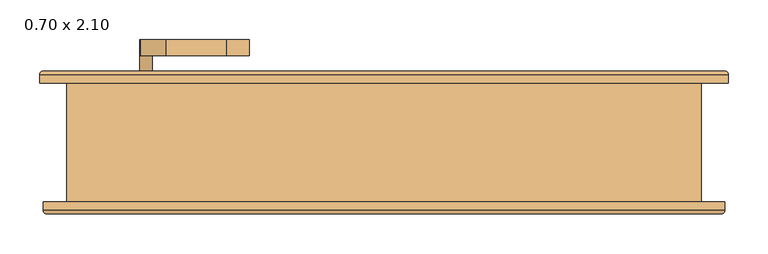
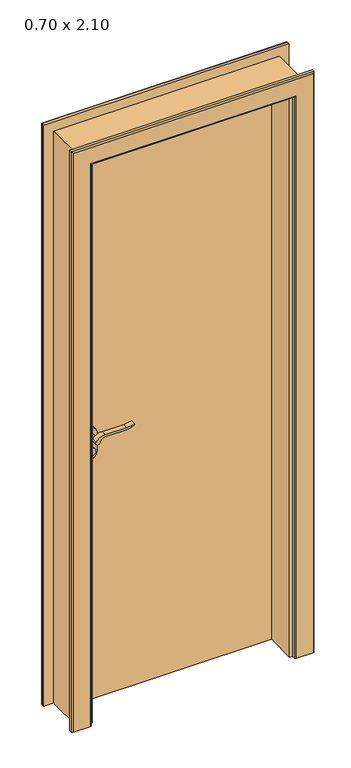
"""IFC4 building model written with IfcOpenShell, lengths in millimetres: door geometry, PORTA_DE_ABRIR_MADEIRA : 0.70 x 2.10."""

from ifc_helpers import new_model, si_unit, point, frame, frame_2d, origin, origin_with_axes, place, context, project, spatial, polyline, circle_curve, ellipse_curve, trimmed, segment, composite_curve, outline, extrude, faceted_brep, source, transform, mapped, element, save
from ifc_brep_helpers import plane_surface, cylinder_surface, advanced_brep


def door_0_70_x_2_10_357bc0c5(model_context):
    return source(origin(), model_context, "Body", "SolidModel", [
        extrude(outline(composite_curve([segment(trimmed(circle_curve(frame_2d((940.0, -300.0)), 15.0), [point((940.0, -285.0))], [point((940.0, -315.0))], False, "CARTESIAN"), True, "CONTINUOUS"), segment(trimmed(circle_curve(frame_2d((940.0, -300.0)), 15.0), [point((940.0, -315.0))], [point((940.0, -285.0))], False, "CARTESIAN"), True, "CONTINUOUS")], self_intersect=False)), frame((0.0, 15.0, 0.0), z_axis=(0.0, 1.0, 0.0), x_axis=(0.0, 0.0, 1.0)), (0.0, 0.0, 1.0), 10.0),
        extrude(outline(composite_curve([segment(trimmed(circle_curve(frame_2d((940.0, -300.0)), 15.0), [point((940.0, -285.0))], [point((940.0, -315.0))], False, "CARTESIAN"), True, "CONTINUOUS"), segment(trimmed(circle_curve(frame_2d((940.0, -300.0)), 15.0), [point((940.0, -315.0))], [point((940.0, -285.0))], False, "CARTESIAN"), True, "CONTINUOUS")], self_intersect=False)), frame((0.0, 80.0, 0.0), z_axis=(0.0, 1.0, 0.0), x_axis=(0.0, 0.0, 1.0)), (0.0, 0.0, 1.0), 10.0),
        extrude(outline(composite_curve([segment(trimmed(circle_curve(frame_2d((1000.0, -300.0)), 8.0), [point((1004.6523287, -306.5081363))], [point((1000.0, -292.0))], False, "CARTESIAN"), True, "CONTINUOUS"), segment(trimmed(circle_curve(frame_2d((994.8738613, -274.6138099)), 18.1261387), [point((1000.0, -292.0))], [point((1013.0, -274.6138099))], True, "CARTESIAN"), True, "CONTINUOUS"), segment(polyline([(1013.0, -274.6138099), (1013.0, -198.3564091)]), True, "CONTINUOUS"), segment(trimmed(circle_curve(frame_2d((1072.2709207, -201.9396612)), 59.3791355), [point((1013.0, -198.3564091))], [point((1022.2135558, -170.0))], False, "CARTESIAN"), True, "CONTINUOUS"), segment(polyline([(1022.2135558, -170.0), (1025.0, -170.0)]), True, "CONTINUOUS"), segment(trimmed(circle_curve(frame_2d((1103.2850638, -198.4227909)), 83.2850902), [point((1025.0, -170.0))], [point((1020.0, -198.3564091))], True, "CARTESIAN"), True, "CONTINUOUS"), segment(polyline([(1020.0, -198.3564091), (1020.0, -274.6325667)]), True, "CONTINUOUS"), segment(trimmed(circle_curve(frame_2d((982.7555521, -276.3324871)), 37.2832219), [point((1020.0, -274.6325667))], [point((1004.6523287, -306.5081363))], False, "CARTESIAN"), True, "CONTINUOUS")], self_intersect=False)), frame((0.0, -25.0, 0.0), z_axis=(0.0, 1.0, 0.0), x_axis=(0.0, 0.0, 1.0)), (0.0, 0.0, 1.0), 20.0),
        extrude(outline(composite_curve([segment(trimmed(circle_curve(frame_2d((994.8738682, -274.6138122)), 18.1261318), [point((999.9999903, -292.0))], [point((1013.0, -274.6138122))], True, "CARTESIAN"), True, "CONTINUOUS"), segment(polyline([(1013.0, -274.6138122), (1013.0, -198.3564091)]), True, "CONTINUOUS"), segment(trimmed(circle_curve(frame_2d((1072.2709207, -201.9396612)), 59.3791355), [point((1013.0, -198.3564091))], [point((1022.2135558, -170.0))], False, "CARTESIAN"), True, "CONTINUOUS"), segment(polyline([(1022.2135558, -170.0), (1025.0, -170.0)]), True, "CONTINUOUS"), segment(trimmed(circle_curve(frame_2d((1103.2850638, -198.4227909)), 83.2850902), [point((1025.0, -170.0))], [point((1020.0, -198.3564091))], True, "CARTESIAN"), True, "CONTINUOUS"), segment(polyline([(1020.0, -198.3564091), (1020.0, -274.6325667)]), True, "CONTINUOUS"), segment(trimmed(circle_curve(frame_2d((982.7555521, -276.3324871)), 37.2832219), [point((1020.0, -274.6325667))], [point((1004.6523287, -306.5081363))], False, "CARTESIAN"), True, "CONTINUOUS"), segment(trimmed(circle_curve(frame_2d((1000.0, -300.0)), 8.0), [point((1004.6523287, -306.5081363))], [point((999.9999903, -292.0))], False, "CARTESIAN"), True, "CONTINUOUS")], self_intersect=False)), frame((0.0, 110.0, 0.0), z_axis=(0.0, 1.0, 0.0), x_axis=(0.0, 0.0, 1.0)), (0.0, 0.0, 1.0), 20.0),
        extrude(outline(composite_curve([segment(trimmed(circle_curve(frame_2d((1000.0, -300.0)), 8.0), [point((1000.0, -292.0))], [point((1000.0, -308.0))], False, "CARTESIAN"), True, "CONTINUOUS"), segment(trimmed(circle_curve(frame_2d((1000.0, -300.0)), 8.0), [point((1000.0, -308.0))], [point((1000.0, -292.0))], False, "CARTESIAN"), True, "CONTINUOUS")], self_intersect=False)), frame((0.0, -5.0, 0.0), z_axis=(0.0, 1.0, 0.0), x_axis=(0.0, 0.0, 1.0)), (0.0, 0.0, 1.0), 30.0),
        extrude(outline(composite_curve([segment(trimmed(circle_curve(frame_2d((1000.0, -300.0)), 8.0), [point((1000.0, -292.0))], [point((1000.0, -308.0))], False, "CARTESIAN"), True, "CONTINUOUS"), segment(trimmed(circle_curve(frame_2d((1000.0, -300.0)), 8.0), [point((1000.0, -308.0))], [point((1000.0, -292.0))], False, "CARTESIAN"), True, "CONTINUOUS")], self_intersect=False)), frame((0.0, 80.0, 0.0), z_axis=(0.0, 1.0, 0.0), x_axis=(0.0, 0.0, 1.0)), (0.0, 0.0, 1.0), 30.0),
        extrude(outline(composite_curve([segment(trimmed(circle_curve(frame_2d((930.0, -300.0)), 25.0), [point((930.0, -325.0))], [point((930.0, -275.0))], False, "CARTESIAN"), True, "CONTINUOUS"), segment(polyline([(930.0, -275.0), (1000.0, -275.0)]), True, "CONTINUOUS"), segment(trimmed(circle_curve(frame_2d((1000.0, -300.0)), 25.0), [point((1000.0, -275.0))], [point((1000.0, -325.0))], False, "CARTESIAN"), True, "CONTINUOUS"), segment(polyline([(1000.0, -325.0), (930.0, -325.0)]), True, "CONTINUOUS")], self_intersect=False)), frame((0.0, 25.0, 0.0), z_axis=(0.0, 1.0, 0.0), x_axis=(0.0, 0.0, 1.0)), (0.0, 0.0, 1.0), 10.0),
        extrude(outline(composite_curve([segment(trimmed(circle_curve(frame_2d((930.0, -300.0)), 25.0), [point((930.0, -325.0))], [point((930.0, -275.0))], False, "CARTESIAN"), True, "CONTINUOUS"), segment(polyline([(930.0, -275.0), (1000.0, -275.0)]), True, "CONTINUOUS"), segment(trimmed(circle_curve(frame_2d((1000.0, -300.0)), 25.0), [point((1000.0, -275.0))], [point((1000.0, -325.0))], False, "CARTESIAN"), True, "CONTINUOUS"), segment(polyline([(1000.0, -325.0), (930.0, -325.0)]), True, "CONTINUOUS")], self_intersect=False)), frame((0.0, 70.0, 0.0), z_axis=(0.0, 1.0, 0.0), x_axis=(0.0, 0.0, 1.0)), (0.0, 0.0, 1.0), 10.0),
        faceted_brep([(-360.0, 35.0, 0.0), (-350.0, 35.0, 0.0), (-350.0, -75.0, 0.0), (-400.0, -75.0, 0.0), (-400.0, 75.0, 0.0), (-360.0, 75.0, 0.0), (-360.0, 75.0, 2100.0), (-360.0, 35.0, 2100.0), (-400.0, 75.0, 2140.0), (400.0, 75.0, 2140.0), (400.0, 75.0, 0.0), (360.0, 75.0, 0.0), (360.0, 75.0, 2100.0), (-400.0, -75.0, 2140.0), (-350.0, -75.0, 2090.0), (350.0, -75.0, 2090.0), (350.0, -75.0, 0.0), (400.0, -75.0, 0.0), (400.0, -75.0, 2140.0), (-350.0, 35.0, 2090.0), (360.0, 35.0, 2100.0), (360.0, 35.0, 0.0), (350.0, 35.0, 0.0), (350.0, 35.0, 2090.0)], [[[0, 1, 2, 3, 4, 5]], [[5, 6, 7, 0]], [[4, 8, 9, 10, 11, 12, 6, 5]], [[3, 13, 8, 4]], [[2, 14, 15, 16, 17, 18, 13, 3]], [[1, 19, 14, 2]], [[0, 7, 20, 21, 22, 23, 19, 1]], [[23, 22, 16, 15]], [[21, 11, 10, 17, 16, 22]], [[12, 11, 21, 20]], [[18, 17, 10, 9]], [[13, 18, 9, 8]], [[19, 23, 15, 14]], [[6, 12, 20, 7]]]),
        advanced_brep(
        [(-430.0, -75.3, 0.0), (-360.0, -75.3, 0.0), (-360.0, -85.3, 0.0), (-365.0, -90.3, 0.0), (-425.0, -90.3, 0.0), (-430.0, -85.3, 0.0), (-430.0, -85.3, 2170.0), (-430.0, -75.3, 2170.0), (-425.0, -90.3, 2165.0), (-365.0, -90.3, 2105.0), (365.0, -90.3, 2105.0), (365.0, -90.3, 0.0), (425.0, -90.3, 0.0), (425.0, -90.3, 2165.0), (-360.0, -85.3, 2100.0), (-360.0, -75.3, 2100.0), (430.0, -75.3, 2170.0), (430.0, -75.3, 0.0), (360.0, -75.3, 0.0), (360.0, -75.3, 2100.0), (430.0, -85.3, 0.0), (360.0, -85.3, 0.0), (360.0, -85.3, 2100.0), (430.0, -85.3, 2170.0)],
        [
            (0, 1),
            (1, 2),
            (2, 3, circle_curve(frame((-365.0, -85.3, 0.0), z_axis=(0.0, 0.0, -1.0), x_axis=(-1.0, 0.0, 0.0)), 5.0)),
            (3, 4),
            (4, 5, circle_curve(frame((-425.0, -85.3, 0.0), z_axis=(0.0, 0.0, -1.0), x_axis=(-1.0, 0.0, 0.0)), 5.0)),
            (5, 0),
            (5, 6),
            (6, 7),
            (7, 0),
            (4, 8),
            (8, 6, ellipse_curve(frame((-425.0, -85.3, 2165.0), z_axis=(-0.7071067811865475, 0.0, -0.7071067811865475), x_axis=(0.7071067811865474, 0.0, -0.7071067811865476)), 7.0710678, 5.0)),
            (3, 9),
            (9, 10),
            (10, 11),
            (11, 12),
            (12, 13),
            (13, 8),
            (2, 14),
            (14, 9, ellipse_curve(frame((-365.0, -85.3, 2105.0), z_axis=(-0.7071067811865475, 0.0, -0.7071067811865475), x_axis=(0.7071067811865474, 0.0, -0.7071067811865476)), 7.0710678, 5.0)),
            (1, 15),
            (15, 14),
            (7, 16),
            (16, 17),
            (17, 18),
            (18, 19),
            (19, 15),
            (17, 20),
            (20, 12, circle_curve(frame((425.0, -85.3, 0.0), z_axis=(0.0, 0.0, -1.0), x_axis=(1.0, 0.0, 0.0)), 5.0)),
            (11, 21, circle_curve(frame((365.0, -85.3, 0.0), z_axis=(0.0, 0.0, -1.0), x_axis=(1.0, 0.0, 0.0)), 5.0)),
            (21, 18),
            (21, 22),
            (22, 19),
            (10, 22, ellipse_curve(frame((365.0, -85.3, 2105.0), z_axis=(0.7071067811865475, 0.0, -0.7071067811865475), x_axis=(0.7071067811865474, 0.0, 0.7071067811865476)), 7.0710678, 5.0)),
            (20, 23),
            (23, 13, ellipse_curve(frame((425.0, -85.3, 2165.0), z_axis=(0.7071067811865475, 0.0, -0.7071067811865475), x_axis=(0.7071067811865474, 0.0, 0.7071067811865476)), 7.0710678, 5.0)),
            (16, 23),
            (6, 23),
            (22, 14),
        ],
        [
            plane_surface(frame((-400.0, 75.0, 0.0), z_axis=(0.0, 0.0, -1.0), x_axis=(0.0, 1.0, 0.0))),
            plane_surface(frame((-430.0, -75.3, 0.0), z_axis=(-1.0, 0.0, 0.0), x_axis=(0.0, 0.0, 1.0))),
            cylinder_surface(frame((-425.0, -85.3, 0.0), z_axis=(0.0, 0.0, -1.0), x_axis=(-1.0, 0.0, 0.0)), 5.0),
            plane_surface(frame((-425.0, -90.3, 0.0), z_axis=(0.0, -1.0, 0.0), x_axis=(0.0, 0.0, 1.0))),
            cylinder_surface(frame((-365.0, -85.3, 0.0), z_axis=(0.0, 0.0, -1.0), x_axis=(-1.0, 0.0, 0.0)), 5.0),
            plane_surface(frame((-360.0, -85.3, 0.0), z_axis=(1.0, 0.0, 0.0), x_axis=(0.0, 0.0, 1.0))),
            plane_surface(frame((-360.0, -75.3, 0.0), z_axis=(0.0, 1.0, 0.0), x_axis=(0.0, 0.0, 1.0))),
            plane_surface(frame((400.0, 75.0, 0.0), z_axis=(0.0, 0.0, -1.0), x_axis=(0.0, 1.0, 0.0))),
            plane_surface(frame((360.0, -85.3, 2100.0), z_axis=(-1.0, 0.0, 0.0), x_axis=(0.0, 0.0, -1.0))),
            cylinder_surface(frame((365.0, -85.3, 2140.0), z_axis=(0.0, 0.0, 1.0), x_axis=(1.0, 0.0, 0.0)), 5.0),
            cylinder_surface(frame((425.0, -85.3, 2140.0), z_axis=(0.0, 0.0, 1.0), x_axis=(1.0, 0.0, 0.0)), 5.0),
            plane_surface(frame((430.0, -75.3, 2170.0), z_axis=(1.0, 0.0, 0.0), x_axis=(0.0, 0.0, -1.0))),
            plane_surface(frame((-430.0, -75.3, 2170.0), z_axis=(0.0, 0.0, 1.0), x_axis=(1.0, 0.0, 0.0))),
            plane_surface(frame((-360.0, -85.3, 2100.0), z_axis=(0.0, 0.0, -1.0), x_axis=(1.0, 0.0, 0.0))),
            cylinder_surface(frame((-400.0, -85.3, 2165.0), z_axis=(-1.0, 0.0, 0.0), x_axis=(0.0, 0.0, 1.0)), 5.0),
            cylinder_surface(frame((-400.0, -85.3, 2105.0), z_axis=(-1.0, 0.0, 0.0), x_axis=(0.0, 0.0, 1.0)), 5.0),
        ],
        [
            (0, [[1, 2, 3, 4, 5, 6]]),
            (1, [[7, 8, 9, -6]]),
            (2, [[10, 11, -7, -5]]),
            (3, [[12, 13, 14, 15, 16, 17, -10, -4]]),
            (4, [[18, 19, -12, -3]]),
            (5, [[20, 21, -18, -2]]),
            (6, [[-9, 22, 23, 24, 25, 26, -20, -1]]),
            (7, [[27, 28, -15, 29, 30, -24]]),
            (8, [[-25, -30, 31, 32]]),
            (9, [[-31, -29, -14, 33]]),
            (10, [[-16, -28, 34, 35]]),
            (11, [[-34, -27, -23, 36]]),
            (12, [[37, -36, -22, -8]]),
            (13, [[-26, -32, 38, -21]]),
            (14, [[-17, -35, -37, -11]]),
            (15, [[-38, -33, -13, -19]]),
        ],
    ),
        advanced_brep(
        [(-429.3155593, 90.2647517, 0.0), (-369.3155593, 90.2647517, 0.0), (-364.3155593, 85.2647517, 0.0), (-364.3155593, 75.2647517, 0.0), (-434.3155593, 75.2647517, 0.0), (-434.3155593, 85.2647517, 0.0), (-434.3155593, 85.2647517, 2174.3155593), (-429.3155593, 90.2647517, 2169.3155593), (-434.3155593, 75.2647517, 2174.3155593), (-364.3155593, 75.2647517, 2104.3155593), (364.3155593, 75.2647517, 2104.3155593), (364.3155593, 75.2647517, 0.0), (434.3155593, 75.2647517, 0.0), (434.3155593, 75.2647517, 2174.3155593), (-364.3155593, 85.2647517, 2104.3155593), (-369.3155593, 90.2647517, 2109.3155593), (429.3155593, 90.2647517, 2169.3155593), (429.3155593, 90.2647517, 0.0), (369.3155593, 90.2647517, 0.0), (369.3155593, 90.2647517, 2109.3155593), (434.3155593, 85.2647517, 0.0), (364.3155593, 85.2647517, 0.0), (364.3155593, 85.2647517, 2104.3155593), (434.3155593, 85.2647517, 2174.3155593)],
        [
            (0, 1),
            (1, 2, circle_curve(frame((-369.3155593, 85.2647517, 0.0), z_axis=(0.0, 0.0, -1.0), x_axis=(-1.0, 0.0, 0.0)), 5.0)),
            (2, 3),
            (3, 4),
            (4, 5),
            (5, 0, circle_curve(frame((-429.3155593, 85.2647517, 0.0), z_axis=(0.0, 0.0, -1.0), x_axis=(-1.0, 0.0, 0.0)), 5.0)),
            (5, 6),
            (6, 7, ellipse_curve(frame((-429.3155593, 85.2647517, 2169.3155593), z_axis=(-0.7071067811865475, 0.0, -0.7071067811865475), x_axis=(0.7071067811865474, 0.0, -0.7071067811865476)), 7.0710678, 5.0)),
            (7, 0),
            (4, 8),
            (8, 6),
            (3, 9),
            (9, 10),
            (10, 11),
            (11, 12),
            (12, 13),
            (13, 8),
            (2, 14),
            (14, 9),
            (1, 15),
            (15, 14, ellipse_curve(frame((-369.3155593, 85.2647517, 2109.3155593), z_axis=(-0.7071067811865475, 0.0, -0.7071067811865475), x_axis=(0.7071067811865474, 0.0, -0.7071067811865476)), 7.0710678, 5.0)),
            (7, 16),
            (16, 17),
            (17, 18),
            (18, 19),
            (19, 15),
            (17, 20, circle_curve(frame((429.3155593, 85.2647517, 0.0), z_axis=(0.0, 0.0, -1.0), x_axis=(1.0, 0.0, 0.0)), 5.0)),
            (20, 12),
            (11, 21),
            (21, 18, circle_curve(frame((369.3155593, 85.2647517, 0.0), z_axis=(0.0, 0.0, -1.0), x_axis=(1.0, 0.0, 0.0)), 5.0)),
            (21, 22),
            (22, 19, ellipse_curve(frame((369.3155593, 85.2647517, 2109.3155593), z_axis=(0.7071067811865475, 0.0, -0.7071067811865475), x_axis=(0.7071067811865474, 0.0, 0.7071067811865476)), 7.0710678, 5.0)),
            (10, 22),
            (20, 23),
            (23, 13),
            (16, 23, ellipse_curve(frame((429.3155593, 85.2647517, 2169.3155593), z_axis=(0.7071067811865475, 0.0, -0.7071067811865475), x_axis=(0.7071067811865474, 0.0, 0.7071067811865476)), 7.0710678, 5.0)),
            (23, 6),
            (14, 22),
        ],
        [
            plane_surface(frame((-400.0, 75.0, 0.0), z_axis=(0.0, 0.0, -1.0), x_axis=(0.0, 1.0, 0.0))),
            cylinder_surface(frame((-429.3155593, 85.2647517, 0.0), z_axis=(0.0, 0.0, -1.0), x_axis=(-1.0, 0.0, 0.0)), 5.0),
            plane_surface(frame((-434.3155593, 85.2647517, 0.0), z_axis=(-1.0, 0.0, 0.0), x_axis=(0.0, 0.0, 1.0))),
            plane_surface(frame((-434.3155593, 75.2647517, 0.0), z_axis=(0.0, -1.0, 0.0), x_axis=(0.0, 0.0, 1.0))),
            plane_surface(frame((-364.3155593, 75.2647517, 0.0), z_axis=(1.0, 0.0, 0.0), x_axis=(0.0, 0.0, 1.0))),
            cylinder_surface(frame((-369.3155593, 85.2647517, 0.0), z_axis=(0.0, 0.0, -1.0), x_axis=(-1.0, 0.0, 0.0)), 5.0),
            plane_surface(frame((-369.3155593, 90.2647517, 0.0), z_axis=(0.0, 1.0, 0.0), x_axis=(0.0, 0.0, 1.0))),
            plane_surface(frame((400.0, 75.0, 0.0), z_axis=(0.0, 0.0, -1.0), x_axis=(0.0, 1.0, 0.0))),
            cylinder_surface(frame((369.3155593, 85.2647517, 2140.0), z_axis=(0.0, 0.0, 1.0), x_axis=(1.0, 0.0, 0.0)), 5.0),
            plane_surface(frame((364.3155593, 75.2647517, 2104.3155593), z_axis=(-1.0, 0.0, 0.0), x_axis=(0.0, 0.0, -1.0))),
            plane_surface(frame((434.3155593, 85.2647517, 2174.3155593), z_axis=(1.0, 0.0, 0.0), x_axis=(0.0, 0.0, -1.0))),
            cylinder_surface(frame((429.3155593, 85.2647517, 2140.0), z_axis=(0.0, 0.0, 1.0), x_axis=(1.0, 0.0, 0.0)), 5.0),
            plane_surface(frame((-434.3155593, 85.2647517, 2174.3155593), z_axis=(0.0, 0.0, 1.0), x_axis=(1.0, 0.0, 0.0))),
            plane_surface(frame((-364.3155593, 75.2647517, 2104.3155593), z_axis=(0.0, 0.0, -1.0), x_axis=(1.0, 0.0, 0.0))),
            cylinder_surface(frame((-400.0, 85.2647517, 2169.3155593), z_axis=(-1.0, 0.0, 0.0), x_axis=(0.0, 0.0, 1.0)), 5.0),
            cylinder_surface(frame((-400.0, 85.2647517, 2109.3155593), z_axis=(-1.0, 0.0, 0.0), x_axis=(0.0, 0.0, 1.0)), 5.0),
        ],
        [
            (0, [[1, 2, 3, 4, 5, 6]]),
            (1, [[7, 8, 9, -6]]),
            (2, [[10, 11, -7, -5]]),
            (3, [[12, 13, 14, 15, 16, 17, -10, -4]]),
            (4, [[18, 19, -12, -3]]),
            (5, [[20, 21, -18, -2]]),
            (6, [[-9, 22, 23, 24, 25, 26, -20, -1]]),
            (7, [[27, 28, -15, 29, 30, -24]]),
            (8, [[-25, -30, 31, 32]]),
            (9, [[-31, -29, -14, 33]]),
            (10, [[-16, -28, 34, 35]]),
            (11, [[-34, -27, -23, 36]]),
            (12, [[-17, -35, 37, -11]]),
            (13, [[38, -33, -13, -19]]),
            (14, [[-37, -36, -22, -8]]),
            (15, [[-26, -32, -38, -21]]),
        ],
    ),
        extrude(outline(polyline([(360.0, 70.0), (360.0, 35.0), (-360.0, 35.0), (-360.0, 70.0), (360.0, 70.0)])), origin_with_axes(), (0.0, 0.0, 1.0), 2100.0),
    ])


if __name__ == "__main__":
    model = new_model("IFC4")
    model_context = context("Model", 3, world=origin())
    ifc_project = project(units=[si_unit("LENGTHUNIT", "METRE", prefix="MILLI")], contexts=[model_context])
    site = spatial("IfcSite", under=ifc_project)
    building = spatial("IfcBuilding", under=site)
    placement = place(None, origin())
    door_0_70_x_2_10_shape = door_0_70_x_2_10_357bc0c5(model_context)
    element("IfcDoor", 1, ObjectType="PORTA_DE_ABRIR_MADEIRA : 0.70 x 2.10", at=placement, inside=building, context=model_context, shape_type="MappedRepresentation", body=[
        mapped(door_0_70_x_2_10_shape, transform((0.0, 0.0, 0.0), x_axis=(1.0, 0.0, 0.0), y_axis=(0.0, 1.0, 0.0), z_axis=(0.0, 0.0, 1.0))),
    ])
    save(model, "model.ifc")

# Revit data of these elements
# Project information
#   Project Issue Date = "Data de emissão"
#   Project Status = "Status do projeto"
# Type "PORTA_DE_ABRIR_MADEIRA : 0.70 x 2.10"
#   Type Mark = "P3"
#   Analytic Construction = "<Nenhum>"
#   Rough Width = 0.80 m
#   Projeção da estrutura externa = 0.025 m
#   Projeção da estrutura interna = 0.025 m
#   Largura da estrutura = 0.075 m
#   Rough Height = 2.15 m
#   Height = 2.10 m
#   Width = 0.70 m
#   Soleira [instance default] = no
#   Material do batente = .BATENTE E GUARNIÇÃO
#   Material da maçaneta = .AÇO INOXIDÁVEL ESCOVADO
#   Material da folha da porta = .FOLHA DA PORTA
#   Material da Soleira [instance default] = none
#   Function = (empty or 0)
#   Wall Closure = (empty or 0)
# Element 1 (IfcDoor, "PORTA_DE_ABRIR_MADEIRA : 0.70 x 2.10")
#   Materials on its faces: ".AÇO INOXIDÁVEL ESCOVADO", ".BATENTE E GUARNIÇÃO", ".FOLHA DA PORTA"
# Materials
#   ".BATENTE E GUARNIÇÃO": class "Madeira", colour RGB 215 186 156, transparency 0, Cost = 0
#   ".AÇO INOXIDÁVEL ESCOVADO": class "Metal", colour RGB 189 187 185, transparency 0, Description = "Stainless Steel 18/8, brushed finish", Cost = 0
#   ".FOLHA DA PORTA": class "Madeira", colour RGB 148 119 91, transparency 0, Cost = 0
